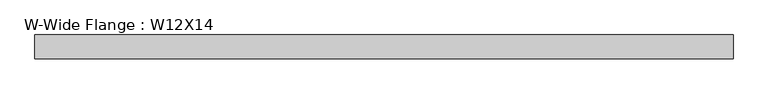
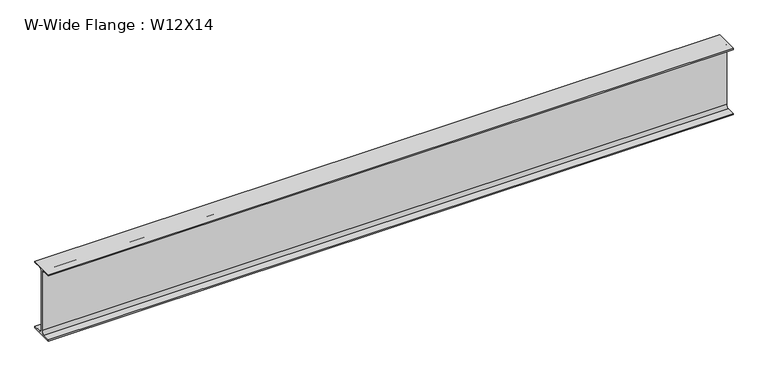
"""IFC4 building model written with IfcOpenShell, lengths in millimetres: beam geometry, W-Wide Flange : W12X14."""

from ifc_helpers import new_model, si_unit, point, frame, frame_2d, origin, place, context, project, spatial, polyline, circle_curve, trimmed, segment, composite_curve, outline, extrude, source, transform, mapped, element, save


def w_wide_flange_w12x14_6311ab4e(model_context):
    return source(origin(), model_context, "Body", "SweptSolid", [
        extrude(outline(composite_curve([segment(polyline([(50.419, -145.415), (50.419, -151.13), (-50.419, -151.13), (-50.419, -145.415), (-15.875, -145.415)]), True, "CONTINUOUS"), segment(trimmed(circle_curve(frame_2d((-15.875, -132.08)), 13.335), [point((-15.875, -145.415))], [point((-2.54, -132.08))], True, "CARTESIAN"), True, "CONTINUOUS"), segment(polyline([(-2.54, -132.08), (-2.54, 132.08)]), True, "CONTINUOUS"), segment(trimmed(circle_curve(frame_2d((-15.875, 132.08)), 13.335), [point((-2.54, 132.08))], [point((-15.875, 145.415))], True, "CARTESIAN"), True, "CONTINUOUS"), segment(polyline([(-15.875, 145.415), (-50.419, 145.415), (-50.419, 151.13), (50.419, 151.13), (50.419, 145.415), (15.875, 145.415)]), True, "CONTINUOUS"), segment(trimmed(circle_curve(frame_2d((15.875, 132.08)), 13.335), [point((15.875, 145.415))], [point((2.54, 132.08))], True, "CARTESIAN"), True, "CONTINUOUS"), segment(polyline([(2.54, 132.08), (2.54, -132.08)]), True, "CONTINUOUS"), segment(trimmed(circle_curve(frame_2d((15.875, -132.08)), 13.335), [point((2.54, -132.08))], [point((15.875, -145.415))], True, "CARTESIAN"), True, "CONTINUOUS"), segment(polyline([(15.875, -145.415), (50.419, -145.415)]), True, "CONTINUOUS")], self_intersect=False)), frame((-1473.2, 0.0, 0.0), z_axis=(1.0, 0.0, 0.0), x_axis=(0.0, 1.0, 0.0)), (0.0, 0.0, 1.0), 2946.4),
    ])


if __name__ == "__main__":
    model = new_model("IFC4")
    model_context = context("Model", 3, world=origin())
    ifc_project = project(units=[si_unit("LENGTHUNIT", "METRE", prefix="MILLI")], contexts=[model_context])
    site = spatial("IfcSite", under=ifc_project)
    building = spatial("IfcBuilding", under=site)
    placement = place(None, origin())
    w_wide_flange_w12x14_shape = w_wide_flange_w12x14_6311ab4e(model_context)
    element("IfcBeam", 1, ObjectType="W-Wide Flange : W12X14", at=placement, inside=building, context=model_context, shape_type="MappedRepresentation", body=[
        mapped(w_wide_flange_w12x14_shape, transform((0.0, 0.0, 0.0), x_axis=(1.0, 0.0, 0.0), y_axis=(0.0, 1.0, 0.0), z_axis=(0.0, 0.0, 1.0))),
    ])
    save(model, "model.ifc")

# Revit data of these elements
# Type "W-Wide Flange : W12X14"
#   Assembly Code = "B10"
#   W = 14
#   Length [instance default] = 5' - 0"
#   bf = 0' - 3.97"
#   d = 0' - 11.9"
#   k = 0' - 0 3/4"
#   k2 = 0' - 0.525"
#   tf = 0' - 0.225"
#   tw = 0' - 0.2"
#   A = 0.0288889 SF
#   Structural Material [instance default] = Steel ASTM A992
# Element 1 (IfcBeam, "W-Wide Flange : W12X14")
#   Materials on its faces: "Steel ASTM A992"
# Materials
#   "Steel ASTM A992": class "Metal", colour RGB 199 199 199, transparency 0, Description = "Structural steel 50ksi", Cost = 0
